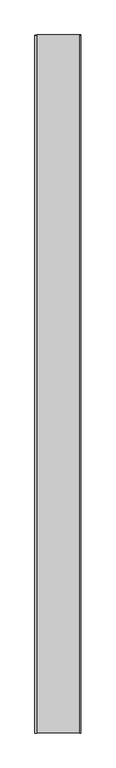
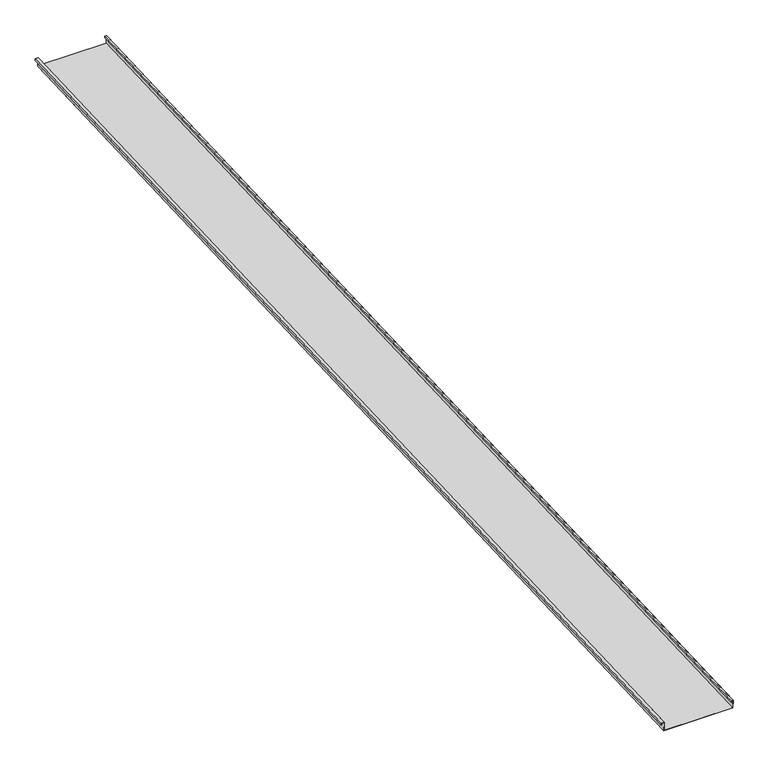
"""IFC4 building model written with IfcOpenShell, lengths in millimetres: proxy geometry, Generic Models 2:Generic Models 2:310765:Generic Models 2:310765 : Generic Models 2:Generic Models 2:310765:123 : Generic Models 2:Generic Models 2:310765:Generic Models 2:310765 : Generic Models 2:Generic Models 2:310765:300385."""

from ifc_helpers import new_model, si_unit, frame, origin, place, context, project, spatial, polyline, outline, extrude, source, transform, mapped, element, save


def generic_models_1f8d129c(model_context):
    return source(origin(), model_context, "Body", "SweptSolid", [
        extrude(outline(polyline([(1.5875, 0.0), (1.5875, 50.8), (407.9875, 50.8), (407.9875, 1.5875), (396.875, 1.5875), (396.875, 11.1125), (398.4625, 11.1125), (398.4625, 3.175), (406.4, 3.175), (406.4, 49.2125), (3.175, 49.2125), (3.175, -1.5874999), (-14.2875, -1.5874999), (-14.2875, 9.525), (-12.7, 9.525), (-12.7, 0.0), (1.5875, 0.0)])), frame((662575.5263072, -581354.4345603, 3902.6697972), z_axis=(0.0, 0.9991330730923568, 0.041630544712067834), x_axis=(1.0, 0.0, 0.0)), (0.0, 0.0, 1.0), 6400.8),
    ])


if __name__ == "__main__":
    model = new_model("IFC4")
    model_context = context("Model", 3, world=origin())
    ifc_project = project(units=[si_unit("LENGTHUNIT", "METRE", prefix="MILLI")], contexts=[model_context])
    site = spatial("IfcSite", under=ifc_project)
    building = spatial("IfcBuilding", under=site)
    placement = place(None, origin())
    generic_models_shape = generic_models_1f8d129c(model_context)
    element("IfcBuildingElementProxy", 1, Name="Generic Models 2:Generic Models 2:310765:Generic Models 2:310765 : Generic Models 2:Generic Models 2:310765:123 : Generic Models 2:Generic Models 2:310765:Generic Models 2:310765 : Generic Models 2:Generic Models 2:310765:300385", ObjectType="Generic Models 2:Generic Models 2:310765:Generic Models 2:310765 : Generic Models 2:Generic Models 2:310765:123 : Generic Models 2:Generic Models 2:310765:Generic Models 2:310765 : Generic Models 2:Generic Models 2:310765:300385", at=placement, inside=building, context=model_context, shape_type="MappedRepresentation", body=[
        mapped(generic_models_shape, transform((0.0, 0.0, 0.0), x_axis=(1.0, 0.0, 0.0), y_axis=(0.0, 1.0, 0.0), z_axis=(0.0, 0.0, 1.0))),
    ])
    save(model, "model.ifc")

# Revit data of these elements
# Type "Generic Models 2:Generic Models 2:310765:Generic Models 2:310765 : Generic Models 2:Generic Models 2:310765:123 : Generic Models 2:Generic Models 2:310765:Generic Models 2:310765 : Generic Models 2:Generic Models 2:310765:300385"
#   NameOverride = "Generic Models 2:Generic Models 2:310765:Generic Models 2:310765 : Generic Models 2:Generic Models 2:310765:300385"
#   ObjectTypeOverride = "Generic Models 2:310765 : Generic Models 2:Generic Models 2:310765"
#   Reference = "Generic Models 2"
#   Tag = "300385"
# Element 1 (IfcBuildingElementProxy, "Generic Models 2:Generic Models 2:310765:Generic Models 2:310765 : Generic Models 2:Generic Models 2:310765:123 : Generic Models 2:Generic Models 2:310765:Generic Models 2:310765 : Generic Models 2:Generic Models 2:310765:300385")
#   Materials on its faces: "THERMAL BROKEN ALUMINUM STOREFRONT FOR POLYCARBONATE"
# Materials
#   "THERMAL BROKEN ALUMINUM STOREFRONT FOR POLYCARBONATE": class "Unassigned", colour RGB 244 244 244, transparency 0, Keynote = "M07611300.01", Cost = 0
